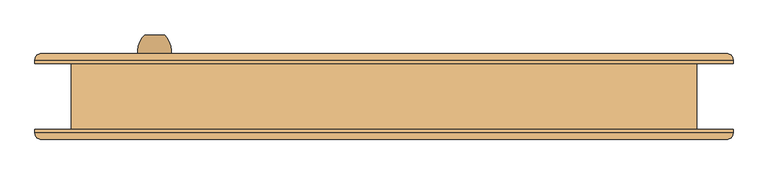
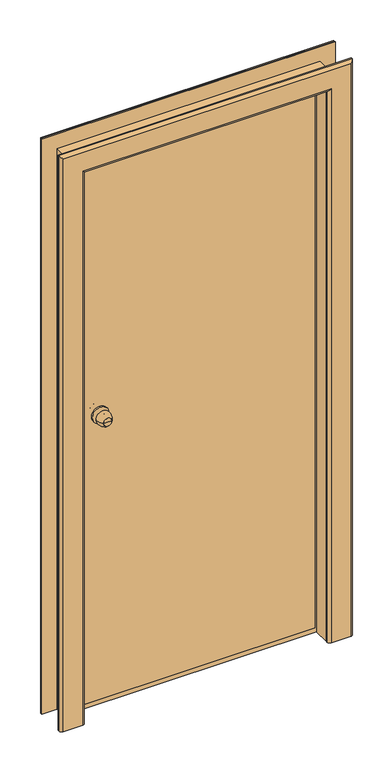
"""IFC4 building model written with IfcOpenShell, lengths in millimetres: door geometry, Наружная дверь 1-Навесная - Один проем наружу с порогом - 31173-2003 : Наружная дверь 1-Навесная - Один проем наружу с порогом - 31173-2003."""

from ifc_helpers import new_model, si_unit, point, frame, origin, place, context, project, spatial, polyline, circle_curve, ellipse_curve, trimmed, outline, extrude, faceted_brep, source, transform, mapped, element, save
from ifc_brep_helpers import plane_surface, cylinder_surface, revolved_surface, advanced_brep


def door_f8daf983(model_context):
    return source(origin(), model_context, "Body", "SolidModel", [
        advanced_brep(
        [(-330.0, 93.0, 1100.0), (-345.0, 93.0, 1100.0), (-360.0, 93.0, 1100.0), (-370.0, 63.0, 1100.0), (-320.0, 63.0, 1100.0), (-363.0, 63.0, 1100.0), (-327.0, 63.0, 1100.0), (-355.0, 55.0, 1100.0), (-335.0, 55.0, 1100.0), (-355.0, 49.0, 1100.0), (-335.0, 49.0, 1100.0), (-375.0, 49.0, 1100.0), (-315.0, 49.0, 1100.0), (-375.0, 43.0, 1100.0), (-315.0, 43.0, 1100.0)],
        [
            (0, 1),
            (1, 2),
            (2, 0, circle_curve(frame((-345.0, 93.0, 1100.0), z_axis=(0.0, 1.0, 0.0), x_axis=(-1.0, 0.0, 0.0)), 15.0)),
            (0, 2, circle_curve(frame((-345.0, 93.0, 1100.0), z_axis=(0.0, 1.0, 0.0), x_axis=(-1.0, 0.0, 0.0)), 15.0)),
            (2, 3, circle_curve(frame((-335.3773735, 68.1257912, 1100.0), z_axis=(0.0, 0.0, 1.0), x_axis=(1.0, 0.0, 0.0)), 35.0)),
            (3, 4, circle_curve(frame((-345.0, 63.0, 1100.0), z_axis=(0.0, 1.0, 0.0), x_axis=(-1.0, 0.0, 0.0)), 25.0)),
            (4, 0, circle_curve(frame((-354.6226265, 68.1257912, 1100.0), z_axis=(0.0, 0.0, 1.0), x_axis=(-1.0, 0.0, 0.0)), 35.0)),
            (4, 3, circle_curve(frame((-345.0, 63.0, 1100.0), z_axis=(0.0, 1.0, 0.0), x_axis=(-1.0, 0.0, 0.0)), 25.0)),
            (3, 5),
            (5, 6, circle_curve(frame((-345.0, 63.0, 1100.0), z_axis=(0.0, 1.0, 0.0), x_axis=(-1.0, 0.0, 0.0)), 18.0)),
            (6, 4),
            (6, 5, circle_curve(frame((-345.0, 63.0, 1100.0), z_axis=(0.0, 1.0, 0.0), x_axis=(-1.0, 0.0, 0.0)), 18.0)),
            (5, 7, circle_curve(frame((-363.0, 55.0, 1100.0), z_axis=(0.0, 0.0, -1.0), x_axis=(1.0, 0.0, 0.0)), 8.0)),
            (7, 8, circle_curve(frame((-345.0, 55.0, 1100.0), z_axis=(0.0, 1.0, 0.0), x_axis=(-1.0, 0.0, 0.0)), 10.0)),
            (8, 6, circle_curve(frame((-327.0, 55.0, 1100.0), z_axis=(0.0, 0.0, -1.0), x_axis=(-1.0, 0.0, 0.0)), 8.0)),
            (8, 7, circle_curve(frame((-345.0, 55.0, 1100.0), z_axis=(0.0, 1.0, 0.0), x_axis=(-1.0, 0.0, 0.0)), 10.0)),
            (7, 9),
            (9, 10, circle_curve(frame((-345.0, 49.0, 1100.0), z_axis=(0.0, 1.0, 0.0), x_axis=(-1.0, 0.0, 0.0)), 10.0)),
            (10, 8),
            (10, 9, circle_curve(frame((-345.0, 49.0, 1100.0), z_axis=(0.0, 1.0, 0.0), x_axis=(-1.0, 0.0, 0.0)), 10.0)),
            (11, 12, circle_curve(frame((-345.0, 49.0, 1100.0), z_axis=(0.0, 1.0, 0.0), x_axis=(1.0, 0.0, 0.0)), 30.0)),
            (12, 11, circle_curve(frame((-345.0, 49.0, 1100.0), z_axis=(0.0, 1.0, 0.0), x_axis=(1.0, 0.0, 0.0)), 30.0)),
            (13, 14, circle_curve(frame((-345.0, 43.0, 1100.0), z_axis=(0.0, -1.0, 0.0), x_axis=(1.0, 0.0, 0.0)), 30.0)),
            (14, 13, circle_curve(frame((-345.0, 43.0, 1100.0), z_axis=(0.0, -1.0, 0.0), x_axis=(1.0, 0.0, 0.0)), 30.0)),
            (12, 14),
            (13, 11),
        ],
        [
            plane_surface(frame((-345.0, 93.0, 1100.0), z_axis=(0.0, 1.0, 0.0), x_axis=(-1.0, 0.0, 0.0))),
            revolved_surface(trimmed(ellipse_curve(frame((-335.3773735, 68.1257912, 1100.0), z_axis=(0.0, 0.0, 1.0), x_axis=(1.0, 0.0, 0.0)), 35.0, 35.0), [point((-360.0, 93.0, 1100.0))], [point((-370.0, 63.0, 1100.0))], True, "CARTESIAN"), (-345.0, 123.0, 1100.0), (0.0, -1.0, 0.0)),
            plane_surface(frame((-345.0, 63.0, 1100.0), z_axis=(0.0, -1.0, 0.0), x_axis=(-1.0, 0.0, 0.0))),
            revolved_surface(trimmed(ellipse_curve(frame((-363.0, 55.0, 1100.0), z_axis=(0.0, 0.0, -1.0), x_axis=(1.0, 0.0, 0.0)), 8.0, 8.0), [point((-363.0, 63.0, 1100.0))], [point((-355.0, 55.0, 1100.0))], True, "CARTESIAN"), (-345.0, 123.0, 1100.0), (0.0, -1.0, 0.0)),
            cylinder_surface(frame((-345.0, 123.0, 1100.0), z_axis=(0.0, -1.0, 0.0), x_axis=(-1.0, 0.0, 0.0)), 10.0),
            plane_surface(frame((-315.0, 49.0, 1100.0), z_axis=(0.0, 1.0, 0.0), x_axis=(0.0, 0.0, 1.0))),
            plane_surface(frame((-315.0, 43.0, 1100.0), z_axis=(0.0, -1.0, 0.0), x_axis=(0.0, 0.0, -1.0))),
            cylinder_surface(frame((-345.0, 43.0, 1100.0), z_axis=(0.0, 1.0, 0.0), x_axis=(1.0, 0.0, 0.0)), 30.0),
        ],
        [
            (0, [[1, 2, 3]]),
            (0, [[-1, 4, -2]]),
            (1, [[5, 6, 7, -3]]),
            (1, [[-7, 8, -5, -4]]),
            (2, [[9, 10, 11, -6]]),
            (2, [[-11, 12, -9, -8]]),
            (3, [[13, 14, 15, -10]]),
            (3, [[-15, 16, -13, -12]]),
            (4, [[17, 18, 19, -14]]),
            (4, [[-19, 20, -17, -16]]),
            (5, [[21, 22], [-20, -18]]),
            (6, [[23, 24]]),
            (7, [[25, -23, 26, -22]]),
            (7, [[-26, -24, -25, -21]]),
        ],
    ),
        advanced_brep(
        [(-360.0, -47.0, 1100.0), (-345.0, -47.0, 1100.0), (-330.0, -47.0, 1100.0), (-320.0, -17.0, 1100.0), (-370.0, -17.0, 1100.0), (-327.0, -17.0, 1100.0), (-363.0, -17.0, 1100.0), (-335.0, -9.0, 1100.0), (-355.0, -9.0, 1100.0), (-335.0, -3.0, 1100.0), (-355.0, -3.0, 1100.0), (-315.0, -3.0, 1100.0), (-375.0, -3.0, 1100.0), (-315.0, 3.0, 1100.0), (-375.0, 3.0, 1100.0)],
        [
            (0, 1),
            (1, 2),
            (2, 0, circle_curve(frame((-345.0, -47.0, 1100.0), z_axis=(0.0, -1.0, 0.0), x_axis=(1.0, 0.0, 0.0)), 15.0)),
            (0, 2, circle_curve(frame((-345.0, -47.0, 1100.0), z_axis=(0.0, -1.0, 0.0), x_axis=(1.0, 0.0, 0.0)), 15.0)),
            (2, 3, circle_curve(frame((-354.6226265, -22.1257912, 1100.0), z_axis=(0.0, 0.0, 1.0), x_axis=(-1.0, 0.0, 0.0)), 35.0)),
            (3, 4, circle_curve(frame((-345.0, -17.0, 1100.0), z_axis=(0.0, -1.0, 0.0), x_axis=(1.0, 0.0, 0.0)), 25.0)),
            (4, 0, circle_curve(frame((-335.3773735, -22.1257912, 1100.0), z_axis=(0.0, 0.0, 1.0), x_axis=(1.0, 0.0, 0.0)), 35.0)),
            (4, 3, circle_curve(frame((-345.0, -17.0, 1100.0), z_axis=(0.0, -1.0, 0.0), x_axis=(1.0, 0.0, 0.0)), 25.0)),
            (3, 5),
            (5, 6, circle_curve(frame((-345.0, -17.0, 1100.0), z_axis=(0.0, -1.0, 0.0), x_axis=(1.0, 0.0, 0.0)), 18.0)),
            (6, 4),
            (6, 5, circle_curve(frame((-345.0, -17.0, 1100.0), z_axis=(0.0, -1.0, 0.0), x_axis=(1.0, 0.0, 0.0)), 18.0)),
            (5, 7, circle_curve(frame((-327.0, -9.0, 1100.0), z_axis=(0.0, 0.0, -1.0), x_axis=(-1.0, 0.0, 0.0)), 8.0)),
            (7, 8, circle_curve(frame((-345.0, -9.0, 1100.0), z_axis=(0.0, -1.0, 0.0), x_axis=(1.0, 0.0, 0.0)), 10.0)),
            (8, 6, circle_curve(frame((-363.0, -9.0, 1100.0), z_axis=(0.0, 0.0, -1.0), x_axis=(1.0, 0.0, 0.0)), 8.0)),
            (8, 7, circle_curve(frame((-345.0, -9.0, 1100.0), z_axis=(0.0, -1.0, 0.0), x_axis=(1.0, 0.0, 0.0)), 10.0)),
            (7, 9),
            (9, 10, circle_curve(frame((-345.0, -3.0, 1100.0), z_axis=(0.0, -1.0, 0.0), x_axis=(1.0, 0.0, 0.0)), 10.0)),
            (10, 8),
            (10, 9, circle_curve(frame((-345.0, -3.0, 1100.0), z_axis=(0.0, -1.0, 0.0), x_axis=(1.0, 0.0, 0.0)), 10.0)),
            (11, 12, circle_curve(frame((-345.0, -3.0, 1100.0), z_axis=(0.0, -1.0, 0.0), x_axis=(-1.0, 0.0, 0.0)), 30.0)),
            (12, 11, circle_curve(frame((-345.0, -3.0, 1100.0), z_axis=(0.0, -1.0, 0.0), x_axis=(-1.0, 0.0, 0.0)), 30.0)),
            (13, 14, circle_curve(frame((-345.0, 3.0, 1100.0), z_axis=(0.0, 1.0, 0.0), x_axis=(-1.0, 0.0, 0.0)), 30.0)),
            (14, 13, circle_curve(frame((-345.0, 3.0, 1100.0), z_axis=(0.0, 1.0, 0.0), x_axis=(-1.0, 0.0, 0.0)), 30.0)),
            (12, 14),
            (13, 11),
        ],
        [
            plane_surface(frame((-345.0, -47.0, 1100.0), z_axis=(0.0, -1.0, 0.0), x_axis=(1.0, 0.0, 0.0))),
            revolved_surface(trimmed(ellipse_curve(frame((-354.6226265, -22.1257912, 1100.0), z_axis=(0.0, 0.0, 1.0), x_axis=(-1.0, 0.0, 0.0)), 35.0, 35.0), [point((-330.0, -47.0, 1100.0))], [point((-320.0, -17.0, 1100.0))], True, "CARTESIAN"), (-345.0, -77.0, 1100.0), (0.0, 1.0, 0.0)),
            plane_surface(frame((-345.0, -17.0, 1100.0), z_axis=(0.0, 1.0, 0.0), x_axis=(1.0, 0.0, 0.0))),
            revolved_surface(trimmed(ellipse_curve(frame((-327.0, -9.0, 1100.0), z_axis=(0.0, 0.0, -1.0), x_axis=(-1.0, 0.0, 0.0)), 8.0, 8.0), [point((-327.0, -17.0, 1100.0))], [point((-335.0, -9.0, 1100.0))], True, "CARTESIAN"), (-345.0, -77.0, 1100.0), (0.0, 1.0, 0.0)),
            cylinder_surface(frame((-345.0, -77.0, 1100.0), z_axis=(0.0, 1.0, 0.0), x_axis=(1.0, 0.0, 0.0)), 10.0),
            plane_surface(frame((-375.0, -3.0, 1100.0), z_axis=(0.0, -1.0, 0.0), x_axis=(0.0, 0.0, 1.0))),
            plane_surface(frame((-375.0, 3.0, 1100.0), z_axis=(0.0, 1.0, 0.0), x_axis=(0.0, 0.0, -1.0))),
            cylinder_surface(frame((-345.0, 3.0, 1100.0), z_axis=(0.0, -1.0, 0.0), x_axis=(-1.0, 0.0, 0.0)), 30.0),
        ],
        [
            (0, [[1, 2, 3]]),
            (0, [[-1, 4, -2]]),
            (1, [[5, 6, 7, -3]]),
            (1, [[-7, 8, -5, -4]]),
            (2, [[9, 10, 11, -6]]),
            (2, [[-11, 12, -9, -8]]),
            (3, [[13, 14, 15, -10]]),
            (3, [[-15, 16, -13, -12]]),
            (4, [[17, 18, 19, -14]]),
            (4, [[-19, 20, -17, -16]]),
            (5, [[21, 22], [-20, -18]]),
            (6, [[23, 24]]),
            (7, [[25, -23, 26, -22]]),
            (7, [[-26, -24, -25, -21]]),
        ],
    ),
        extrude(outline(polyline([(0.0, 470.0), (2120.0, 470.0), (2120.0, -470.0), (0.0, -470.0), (0.0, -450.0), (2100.0, -450.0), (2100.0, 450.0), (0.0, 450.0), (0.0, 470.0)])), frame((0.0, -50.0, 0.0), z_axis=(0.0, 1.0, 0.0), x_axis=(0.0, 0.0, 1.0)), (0.0, 0.0, 1.0), 100.0),
        advanced_brep(
        [(525.0, -50.0, 0.0), (525.0, -55.0, 0.0), (515.0, -65.0, 0.0), (445.0, -65.0, 0.0), (435.0, -55.0, 0.0), (435.0, -50.0, 0.0), (435.0, -50.0, 2085.0), (-435.0, -50.0, 2085.0), (-435.0, -50.0, 0.0), (-525.0, -50.0, 0.0), (-525.0, -50.0, 2175.0), (525.0, -50.0, 2175.0), (435.0, -55.0, 2085.0), (445.0, -65.0, 2095.0), (515.0, -65.0, 2165.0), (-515.0, -65.0, 2165.0), (-515.0, -65.0, 0.0), (-445.0, -65.0, 0.0), (-445.0, -65.0, 2095.0), (525.0, -55.0, 2175.0), (-525.0, -55.0, 0.0), (-525.0, -55.0, 2175.0), (-435.0, -55.0, 0.0), (-435.0, -55.0, 2085.0)],
        [
            (0, 1),
            (1, 2, circle_curve(frame((515.0, -55.0, 0.0), z_axis=(0.0, 0.0, -1.0), x_axis=(1.0, 0.0, 0.0)), 10.0)),
            (2, 3),
            (3, 4, circle_curve(frame((445.0, -55.0, 0.0), z_axis=(0.0, 0.0, -1.0), x_axis=(1.0, 0.0, 0.0)), 10.0)),
            (4, 5),
            (5, 0),
            (5, 6),
            (6, 7),
            (7, 8),
            (8, 9),
            (9, 10),
            (10, 11),
            (11, 0),
            (4, 12),
            (12, 6),
            (3, 13),
            (13, 12, ellipse_curve(frame((445.0, -55.0, 2095.0), z_axis=(0.7071067811865475, 0.0, -0.7071067811865475), x_axis=(-0.7071067811865474, 0.0, -0.7071067811865476)), 14.1421356, 10.0)),
            (2, 14),
            (14, 15),
            (15, 16),
            (16, 17),
            (17, 18),
            (18, 13),
            (1, 19),
            (19, 14, ellipse_curve(frame((515.0, -55.0, 2165.0), z_axis=(0.7071067811865475, 0.0, -0.7071067811865475), x_axis=(-0.7071067811865474, 0.0, -0.7071067811865476)), 14.1421356, 10.0)),
            (11, 19),
            (9, 20),
            (20, 21),
            (21, 10),
            (8, 22),
            (22, 17, circle_curve(frame((-445.0, -55.0, 0.0), z_axis=(0.0, 0.0, -1.0), x_axis=(-1.0, 0.0, 0.0)), 10.0)),
            (16, 20, circle_curve(frame((-515.0, -55.0, 0.0), z_axis=(0.0, 0.0, -1.0), x_axis=(-1.0, 0.0, 0.0)), 10.0)),
            (23, 22),
            (7, 23),
            (23, 18, ellipse_curve(frame((-445.0, -55.0, 2095.0), z_axis=(-0.7071067811865475, 0.0, -0.7071067811865475), x_axis=(-0.7071067811865474, 0.0, 0.7071067811865476)), 14.1421356, 10.0)),
            (15, 21, ellipse_curve(frame((-515.0, -55.0, 2165.0), z_axis=(-0.7071067811865475, 0.0, -0.7071067811865475), x_axis=(-0.7071067811865474, 0.0, 0.7071067811865476)), 14.1421356, 10.0)),
            (12, 23),
            (19, 21),
        ],
        [
            plane_surface(frame((470.0, -50.0, 0.0), z_axis=(0.0, 0.0, -1.0), x_axis=(0.0, 1.0, 0.0))),
            plane_surface(frame((525.0, -50.0, 0.0), z_axis=(0.0, 1.0, 0.0), x_axis=(0.0, 0.0, 1.0))),
            plane_surface(frame((435.0, -50.0, 0.0), z_axis=(-1.0, 0.0, 0.0), x_axis=(0.0, 0.0, 1.0))),
            cylinder_surface(frame((445.0, -55.0, 0.0), z_axis=(0.0, 0.0, -1.0), x_axis=(1.0, 0.0, 0.0)), 10.0),
            plane_surface(frame((445.0, -65.0, 0.0), z_axis=(0.0, -1.0, 0.0), x_axis=(0.0, 0.0, 1.0))),
            cylinder_surface(frame((515.0, -55.0, 0.0), z_axis=(0.0, 0.0, -1.0), x_axis=(1.0, 0.0, 0.0)), 10.0),
            plane_surface(frame((525.0, -55.0, 0.0), z_axis=(1.0, 0.0, 0.0), x_axis=(0.0, 0.0, 1.0))),
            plane_surface(frame((-525.0, -55.0, 2175.0), z_axis=(-1.0, 0.0, 0.0), x_axis=(0.0, 0.0, -1.0))),
            plane_surface(frame((-470.0, -50.0, 0.0), z_axis=(0.0, 0.0, -1.0), x_axis=(0.0, 1.0, 0.0))),
            plane_surface(frame((-435.0, -50.0, 2085.0), z_axis=(1.0, 0.0, 0.0), x_axis=(0.0, 0.0, -1.0))),
            cylinder_surface(frame((-445.0, -55.0, 2120.0), z_axis=(0.0, 0.0, 1.0), x_axis=(-1.0, 0.0, 0.0)), 10.0),
            cylinder_surface(frame((-515.0, -55.0, 2120.0), z_axis=(0.0, 0.0, 1.0), x_axis=(-1.0, 0.0, 0.0)), 10.0),
            plane_surface(frame((435.0, -50.0, 2085.0), z_axis=(0.0, 0.0, -1.0), x_axis=(-1.0, 0.0, 0.0))),
            cylinder_surface(frame((470.0, -55.0, 2095.0), z_axis=(1.0, 0.0, 0.0), x_axis=(0.0, 0.0, 1.0)), 10.0),
            cylinder_surface(frame((470.0, -55.0, 2165.0), z_axis=(1.0, 0.0, 0.0), x_axis=(0.0, 0.0, 1.0)), 10.0),
            plane_surface(frame((525.0, -55.0, 2175.0), z_axis=(0.0, 0.0, 1.0), x_axis=(-1.0, 0.0, 0.0))),
        ],
        [
            (0, [[1, 2, 3, 4, 5, 6]]),
            (1, [[7, 8, 9, 10, 11, 12, 13, -6]]),
            (2, [[14, 15, -7, -5]]),
            (3, [[16, 17, -14, -4]]),
            (4, [[18, 19, 20, 21, 22, 23, -16, -3]]),
            (5, [[24, 25, -18, -2]]),
            (6, [[-13, 26, -24, -1]]),
            (7, [[-11, 27, 28, 29]]),
            (8, [[-10, 30, 31, -21, 32, -27]]),
            (9, [[33, -30, -9, 34]]),
            (10, [[-22, -31, -33, 35]]),
            (11, [[-28, -32, -20, 36]]),
            (12, [[37, -34, -8, -15]]),
            (13, [[-23, -35, -37, -17]]),
            (14, [[38, -36, -19, -25]]),
            (15, [[-12, -29, -38, -26]]),
        ],
    ),
        advanced_brep(
        [(-525.0, 50.0, 0.0), (-525.0, 55.0, 0.0), (-515.0, 65.0, 0.0), (-445.0, 65.0, 0.0), (-435.0, 55.0, 0.0), (-435.0, 50.0, 0.0), (-435.0, 50.0, 2085.0), (435.0, 50.0, 2085.0), (435.0, 50.0, 0.0), (525.0, 50.0, 0.0), (525.0, 50.0, 2175.0), (-525.0, 50.0, 2175.0), (-435.0, 55.0, 2085.0), (-445.0, 65.0, 2095.0), (-515.0, 65.0, 2165.0), (515.0, 65.0, 2165.0), (515.0, 65.0, 0.0), (445.0, 65.0, 0.0), (445.0, 65.0, 2095.0), (-525.0, 55.0, 2175.0), (525.0, 55.0, 0.0), (525.0, 55.0, 2175.0), (435.0, 55.0, 0.0), (435.0, 55.0, 2085.0)],
        [
            (0, 1),
            (1, 2, circle_curve(frame((-515.0, 55.0, 0.0), z_axis=(0.0, 0.0, -1.0), x_axis=(-1.0, 0.0, 0.0)), 10.0)),
            (2, 3),
            (3, 4, circle_curve(frame((-445.0, 55.0, 0.0), z_axis=(0.0, 0.0, -1.0), x_axis=(-1.0, 0.0, 0.0)), 10.0)),
            (4, 5),
            (5, 0),
            (5, 6),
            (6, 7),
            (7, 8),
            (8, 9),
            (9, 10),
            (10, 11),
            (11, 0),
            (4, 12),
            (12, 6),
            (3, 13),
            (13, 12, ellipse_curve(frame((-445.0, 55.0, 2095.0), z_axis=(-0.7071067811865475, 0.0, -0.7071067811865475), x_axis=(0.7071067811865474, 0.0, -0.7071067811865476)), 14.1421356, 10.0)),
            (2, 14),
            (14, 15),
            (15, 16),
            (16, 17),
            (17, 18),
            (18, 13),
            (1, 19),
            (19, 14, ellipse_curve(frame((-515.0, 55.0, 2165.0), z_axis=(-0.7071067811865475, 0.0, -0.7071067811865475), x_axis=(0.7071067811865474, 0.0, -0.7071067811865476)), 14.1421356, 10.0)),
            (11, 19),
            (9, 20),
            (20, 21),
            (21, 10),
            (8, 22),
            (22, 17, circle_curve(frame((445.0, 55.0, 0.0), z_axis=(0.0, 0.0, -1.0), x_axis=(1.0, 0.0, 0.0)), 10.0)),
            (16, 20, circle_curve(frame((515.0, 55.0, 0.0), z_axis=(0.0, 0.0, -1.0), x_axis=(1.0, 0.0, 0.0)), 10.0)),
            (23, 22),
            (7, 23),
            (23, 18, ellipse_curve(frame((445.0, 55.0, 2095.0), z_axis=(0.7071067811865475, 0.0, -0.7071067811865475), x_axis=(0.7071067811865474, 0.0, 0.7071067811865476)), 14.1421356, 10.0)),
            (15, 21, ellipse_curve(frame((515.0, 55.0, 2165.0), z_axis=(0.7071067811865475, 0.0, -0.7071067811865475), x_axis=(0.7071067811865474, 0.0, 0.7071067811865476)), 14.1421356, 10.0)),
            (12, 23),
            (19, 21),
        ],
        [
            plane_surface(frame((-470.0, 50.0, 0.0), z_axis=(0.0, 0.0, -1.0), x_axis=(0.0, 1.0, 0.0))),
            plane_surface(frame((-525.0, 50.0, 0.0), z_axis=(0.0, -1.0, 0.0), x_axis=(0.0, 0.0, 1.0))),
            plane_surface(frame((-435.0, 50.0, 0.0), z_axis=(1.0, 0.0, 0.0), x_axis=(0.0, 0.0, 1.0))),
            cylinder_surface(frame((-445.0, 55.0, 0.0), z_axis=(0.0, 0.0, -1.0), x_axis=(-1.0, 0.0, 0.0)), 10.0),
            plane_surface(frame((-445.0, 65.0, 0.0), z_axis=(0.0, 1.0, 0.0), x_axis=(0.0, 0.0, 1.0))),
            cylinder_surface(frame((-515.0, 55.0, 0.0), z_axis=(0.0, 0.0, -1.0), x_axis=(-1.0, 0.0, 0.0)), 10.0),
            plane_surface(frame((-525.0, 55.0, 0.0), z_axis=(-1.0, 0.0, 0.0), x_axis=(0.0, 0.0, 1.0))),
            plane_surface(frame((525.0, 55.0, 2175.0), z_axis=(1.0, 0.0, 0.0), x_axis=(0.0, 0.0, -1.0))),
            plane_surface(frame((470.0, 50.0, 0.0), z_axis=(0.0, 0.0, -1.0), x_axis=(0.0, 1.0, 0.0))),
            plane_surface(frame((435.0, 50.0, 2085.0), z_axis=(-1.0, 0.0, 0.0), x_axis=(0.0, 0.0, -1.0))),
            cylinder_surface(frame((445.0, 55.0, 2120.0), z_axis=(0.0, 0.0, 1.0), x_axis=(1.0, 0.0, 0.0)), 10.0),
            cylinder_surface(frame((515.0, 55.0, 2120.0), z_axis=(0.0, 0.0, 1.0), x_axis=(1.0, 0.0, 0.0)), 10.0),
            plane_surface(frame((-435.0, 50.0, 2085.0), z_axis=(0.0, 0.0, -1.0), x_axis=(1.0, 0.0, 0.0))),
            cylinder_surface(frame((-470.0, 55.0, 2095.0), z_axis=(-1.0, 0.0, 0.0), x_axis=(0.0, 0.0, 1.0)), 10.0),
            cylinder_surface(frame((-470.0, 55.0, 2165.0), z_axis=(-1.0, 0.0, 0.0), x_axis=(0.0, 0.0, 1.0)), 10.0),
            plane_surface(frame((-525.0, 55.0, 2175.0), z_axis=(0.0, 0.0, 1.0), x_axis=(1.0, 0.0, 0.0))),
        ],
        [
            (0, [[1, 2, 3, 4, 5, 6]]),
            (1, [[7, 8, 9, 10, 11, 12, 13, -6]]),
            (2, [[14, 15, -7, -5]]),
            (3, [[16, 17, -14, -4]]),
            (4, [[18, 19, 20, 21, 22, 23, -16, -3]]),
            (5, [[24, 25, -18, -2]]),
            (6, [[-13, 26, -24, -1]]),
            (7, [[-11, 27, 28, 29]]),
            (8, [[-10, 30, 31, -21, 32, -27]]),
            (9, [[33, -30, -9, 34]]),
            (10, [[-22, -31, -33, 35]]),
            (11, [[-28, -32, -20, 36]]),
            (12, [[37, -34, -8, -15]]),
            (13, [[-23, -35, -37, -17]]),
            (14, [[38, -36, -19, -25]]),
            (15, [[-12, -29, -38, -26]]),
        ],
    ),
        faceted_brep([(450.0, 10.0, 0.0), (-450.0, 10.0, 0.0), (-450.0, 50.0, 0.0), (450.0, 50.0, 0.0), (-450.0, 10.0, 2100.0), (-450.0, 50.0, 2100.0), (450.0, 50.0, 2100.0), (-390.0, 50.0, 2040.0), (-390.0, 50.0, 60.0), (390.0, 50.0, 60.0), (390.0, 50.0, 2040.0), (450.0, 10.0, 2100.0), (-410.0, 10.0, 40.0), (-410.0, 10.0, 2060.0), (410.0, 10.0, 2060.0), (410.0, 10.0, 40.0), (410.0, 45.0, 40.0), (-410.0, 45.0, 40.0), (-410.0, 45.0, 2060.0), (410.0, 45.0, 2060.0), (-390.0, 45.0, 60.0), (-390.0, 45.0, 2040.0), (390.0, 45.0, 2040.0), (390.0, 45.0, 60.0)], [[[0, 1, 2, 3]], [[1, 4, 5, 2]], [[2, 5, 6, 3], [7, 8, 9, 10]], [[4, 1, 0, 11], [12, 13, 14, 15]], [[16, 17, 12, 15]], [[17, 18, 13, 12]], [[18, 17, 16, 19], [20, 21, 22, 23]], [[9, 8, 20, 23]], [[8, 7, 21, 20]], [[11, 0, 3, 6]], [[19, 16, 15, 14]], [[10, 9, 23, 22]], [[4, 11, 6, 5]], [[18, 19, 14, 13]], [[7, 10, 22, 21]]]),
        extrude(outline(polyline([(0.0, 450.0), (2100.0, 450.0), (2100.0, -450.0), (0.0, -450.0), (0.0, -435.0), (2085.0, -435.0), (2085.0, 435.0), (0.0, 435.0), (0.0, 450.0)])), frame((0.0, -50.0, 0.0), z_axis=(0.0, 1.0, 0.0), x_axis=(0.0, 0.0, 1.0)), (0.0, 0.0, 1.0), 60.0),
        faceted_brep([(425.0, 3.0, 22.0), (-425.0, 3.0, 22.0), (-425.0, 8.0, 22.0), (425.0, 8.0, 22.0), (425.0, 3.0, 2075.0), (425.0, 8.0, 2075.0), (-425.0, 8.0, 2075.0), (405.0, 8.0, 2055.0), (-405.0, 8.0, 2055.0), (-405.0, 8.0, 42.0), (405.0, 8.0, 42.0), (-425.0, 3.0, 2075.0), (405.0, 43.0, 42.0), (405.0, 43.0, 2055.0), (-405.0, 43.0, 42.0), (-405.0, 43.0, 2055.0)], [[[0, 1, 2, 3]], [[4, 0, 3, 5]], [[5, 3, 2, 6], [7, 8, 9, 10]], [[2, 1, 11, 6]], [[11, 1, 0, 4]], [[7, 10, 12, 13]], [[9, 14, 12, 10]], [[15, 14, 9, 8]], [[13, 12, 14, 15]], [[4, 5, 6, 11]], [[7, 13, 15, 8]]]),
    ])


if __name__ == "__main__":
    model = new_model("IFC4")
    model_context = context("Model", 3, world=origin())
    ifc_project = project(units=[si_unit("LENGTHUNIT", "METRE", prefix="MILLI")], contexts=[model_context])
    site = spatial("IfcSite", under=ifc_project)
    building = spatial("IfcBuilding", under=site)
    placement = place(None, origin())
    door_shape = door_f8daf983(model_context)
    element("IfcDoor", 1, ObjectType="Наружная дверь 1-Навесная - Один проем наружу с порогом - 31173-2003 : Наружная дверь 1-Навесная - Один проем наружу с порогом - 31173-2003", at=placement, inside=building, context=model_context, shape_type="MappedRepresentation", body=[
        mapped(door_shape, transform((0.0, 0.0, 0.0), x_axis=(1.0, 0.0, 0.0), y_axis=(0.0, 1.0, 0.0), z_axis=(0.0, 0.0, 1.0))),
    ])
    save(model, "model.ifc")

# Revit data of these elements
# Type "Наружная дверь 1-Навесная - Один проем наружу с порогом - 31173-2003 : Наружная дверь 1-Навесная - Один проем наружу с порогом - 31173-2003"
#   Type Mark = "35"
#   Construction Type Id = "MDOOR"
#   Description = "Описание"
#   Analytic Construction = "Металл"
#   Проекционное соединение по ширине = 90 mm
#   Rough Width = 940 mm
#   Rough Height = 2120 mm
#   Угол проема [instance default] = 30.00°
#   Толщина_Тепл_Изоляции = 20 mm
#   Heat Transfer Coefficient (U) = 3.7021 W/(m²·K)
#   Height = 2100 mm
#   Width = 900 mm
#   Ширина каркаса = 40 mm
#   Толщина каркаса = 40 mm
#   Вставка двери [instance default] = 0 mm
#   Define Thermal Properties by = 1
#   Правая сторона = yes
#   Левая сторона = no
#   Function = 1
#   Обрезка = Сталь
#   Панель = Сталь
#   Тепловая изоляция = Тепловая изоляция
#   Кадр = Сталь
#   Дверная ручка = Металл
#   Visual Light Transmittance = 0
#   Solar Heat Gain Coefficient = 0
#   Wall Closure = (empty or 0)
# Element 1 (IfcDoor, "Наружная дверь 1-Навесная - Один проем наружу с порогом - 31173-2003 : Наружная дверь 1-Навесная - Один проем наружу с порогом - 31173-2003")
#   Materials on its faces: "Сталь", "Металл", "Тепловая изоляция"
# Materials
#   "Сталь": class "Металл", colour RGB 247 247 247, transparency 0
#   "Тепловая изоляция": class "Пластмасса", colour RGB 185 154 119, transparency 0
#   "Металл": class "Металл", colour RGB 249 249 249, transparency 0
